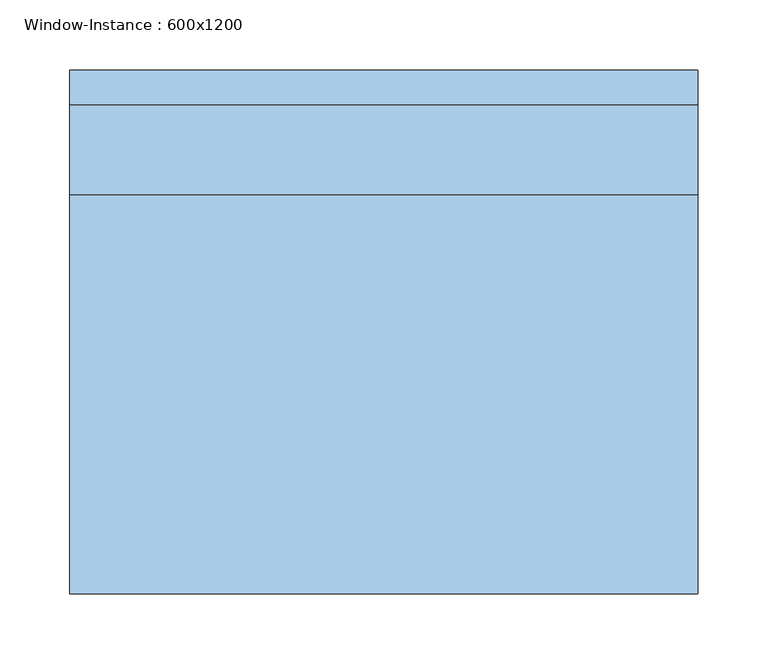
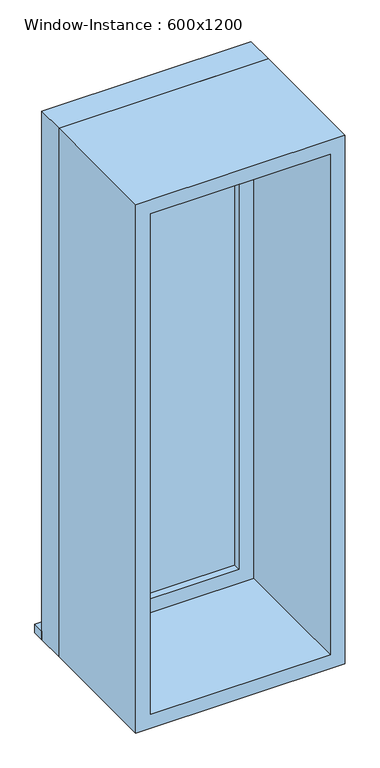
"""IFC4 building model written with IfcOpenShell, lengths in millimetres: window geometry, Window-Instance : 600x1200."""

from ifc_helpers import new_model, si_unit, frame, origin, place, context, project, spatial, polyline, outline, extrude, source, transform, mapped, element, save


def window_instance_600x1200_73f503d8(model_context):
    return source(origin(), model_context, "Body", "SweptSolid", [
        extrude(outline(polyline([(-263.1, 200.4), (186.9, 200.4), (186.9, 175.0), (-263.1, 175.0), (-263.1, 200.4)])), frame((0.0, 0.0, 900.0), z_axis=(0.0, 0.0, 1.0), x_axis=(1.0, 0.0, 0.0)), (0.0, 0.0, 1.0), 19.05),
        extrude(outline(polyline([(123.4, 126.425), (-199.6, 126.425), (-199.6, 139.125), (123.4, 139.125), (123.4, 126.425)])), frame((0.0, 0.0, 963.5), z_axis=(0.0, 0.0, 1.0), x_axis=(1.0, 0.0, 0.0)), (0.0, 0.0, 1.0), 1073.0),
        extrude(outline(polyline([(2080.95, -244.05), (919.05, -244.05), (919.05, 167.85), (2080.95, 167.85), (2080.95, -244.05)]), holes=[polyline([(2036.5, -199.6), (2036.5, 123.4), (963.5, 123.4), (963.5, -199.6), (2036.5, -199.6)])]), frame((0.0, 110.55, 0.0), z_axis=(0.0, 1.0, 0.0), x_axis=(0.0, 0.0, 1.0)), (0.0, 0.0, 1.0), 44.45),
        extrude(outline(polyline([(2100.0, -263.1), (900.0, -263.1), (900.0, 186.9), (2100.0, 186.9), (2100.0, -263.1)]), holes=[polyline([(2068.25, -231.35), (2068.25, 155.15), (931.75, 155.15), (931.75, -231.35), (2068.25, -231.35)])]), frame((0.0, -175.0, 0.0), z_axis=(0.0, 1.0, 0.0), x_axis=(0.0, 0.0, 1.0)), (0.0, 0.0, 1.0), 285.55),
        extrude(outline(polyline([(2100.0, 186.9), (2100.0, -263.1), (900.0, -263.1), (900.0, 186.9), (2100.0, 186.9)]), holes=[polyline([(2080.95, 167.85), (919.05, 167.85), (919.05, -244.05), (2080.95, -244.05), (2080.95, 167.85)])]), frame((0.0, 110.55, 0.0), z_axis=(0.0, 1.0, 0.0), x_axis=(0.0, 0.0, 1.0)), (0.0, 0.0, 1.0), 64.45),
    ])


if __name__ == "__main__":
    model = new_model("IFC4")
    model_context = context("Model", 3, world=origin())
    ifc_project = project(units=[si_unit("LENGTHUNIT", "METRE", prefix="MILLI")], contexts=[model_context])
    site = spatial("IfcSite", under=ifc_project)
    building = spatial("IfcBuilding", under=site)
    placement = place(None, origin())
    window_instance_600x1200_shape = window_instance_600x1200_73f503d8(model_context)
    element("IfcWindow", 1, ObjectType="Window-Instance : 600x1200", at=placement, inside=building, context=model_context, shape_type="MappedRepresentation", body=[
        mapped(window_instance_600x1200_shape, transform((0.0, 0.0, 0.0), x_axis=(1.0, 0.0, 0.0), y_axis=(0.0, 1.0, 0.0), z_axis=(0.0, 0.0, 1.0))),
    ])
    save(model, "model.ifc")

# Revit data of these elements
# Type "Window-Instance : 600x1200"
#   Type Mark = "7"
#   Construction Type Id = "GSP4R"
#   Assembly Code = "B2020100"
#   Analytic Construction = "1/8 in Pilkington single glazing"
#   Visual Light Transmittance = 0.9
#   Thermal Resistance (R) = 0.149095 (m²·K)/W
#   Solar Heat Gain Coefficient = 0.86
#   Heat Transfer Coefficient (U) = 6.70716 W/(m²·K)
#   Height [instance default] = 1200 mm
#   Default Sill Height = 900 mm
#   Width [instance default] = 600 mm
#   Window Inset = 20 mm
#   Glass Pane Material = WW-EC-GL-Storefront
#   Sash Material = WW-EC-RGB-White
#   Wall Closure = (empty or 0)
# Element 1 (IfcWindow, "Window-Instance : 600x1200")
#   Width = 450 mm
#   Materials on its faces: "WW-EC-RGB-White", "WW-EC-GL-Storefront"
# Materials
#   "WW-EC-GL-Storefront": class "Glass", colour RGB 236 240 239, transparency 0.85, Description = "Storefront Glass", Cost = 0
#   "WW-EC-RGB-White": class "Generic", colour RGB 255 255 255, transparency 0, Comments = "If region requests off-white, swith asset color to RGB 231-228-220", Description = "Generic Color", Cost = 0
